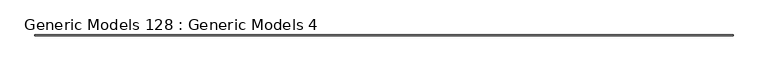
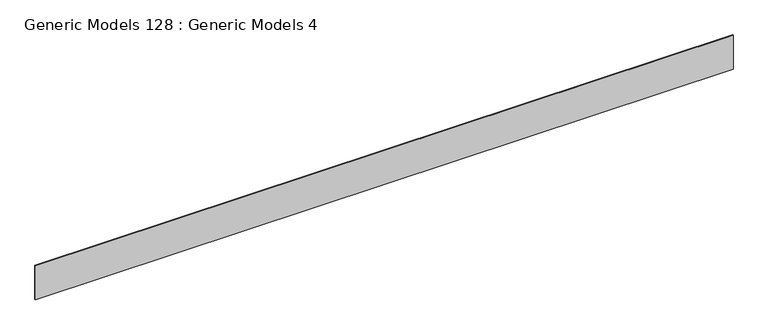
"""IFC4 building model written with IfcOpenShell, lengths in millimetres: proxy geometry, Generic Models 128 : Generic Models 4."""

from ifc_helpers import new_model, si_unit, frame, origin, place, context, project, spatial, polyline, outline, extrude, source, transform, mapped, element, save


def generic_models_128_generic_models_4_9edb3263(model_context):
    return source(origin(), model_context, "Body", "SweptSolid", [
        extrude(outline(polyline([(6870.2180906, 124193.2750923), (6870.2180906, 123243.7809283), (6851.0769662, 123237.6284241), (6851.0769662, 124193.2750923), (6870.2180906, 124193.2750923)])), frame((-10234.5171316, 0.0, 0.0), z_axis=(1.0, 0.0, 0.0), x_axis=(0.0, 1.0, 0.0)), (0.0, 0.0, 1.0), 18643.6),
    ])


if __name__ == "__main__":
    model = new_model("IFC4")
    model_context = context("Model", 3, world=origin())
    ifc_project = project(units=[si_unit("LENGTHUNIT", "METRE", prefix="MILLI")], contexts=[model_context])
    site = spatial("IfcSite", under=ifc_project)
    building = spatial("IfcBuilding", under=site)
    placement = place(None, origin())
    generic_models_128_generic_models_4_shape = generic_models_128_generic_models_4_9edb3263(model_context)
    element("IfcBuildingElementProxy", 1, Name="Generic Models 128 : Generic Models 4", ObjectType="Generic Models 128 : Generic Models 4", at=placement, inside=building, context=model_context, shape_type="MappedRepresentation", body=[
        mapped(generic_models_128_generic_models_4_shape, transform((0.0, 0.0, 0.0), x_axis=(1.0, 0.0, 0.0), y_axis=(0.0, 1.0, 0.0), z_axis=(0.0, 0.0, 1.0))),
    ])
    save(model, "model.ifc")

# Revit data of these elements
# Element 1 (IfcBuildingElementProxy, "Generic Models 128 : Generic Models 4")
#   Materials on its faces: "_7/8\" SMOOTH TROWEL EXTERIOR STUCCO (COLOR PER OWNER)"
# Materials
#   "_7/8\" SMOOTH TROWEL EXTERIOR STUCCO (COLOR PER OWNER)": class "Generic", colour RGB 233 233 233, transparency 0, Cost = 0
